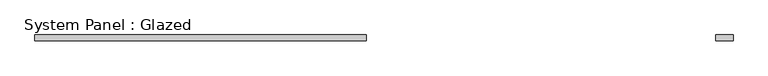
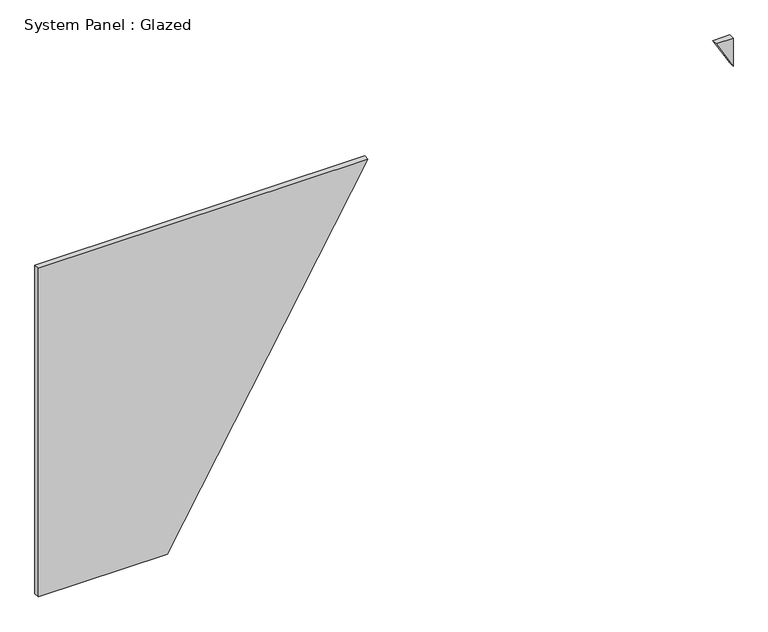
"""IFC4 building model written with IfcOpenShell, lengths in millimetres: plate geometry, System Panel : Glazed."""

from ifc_helpers import new_model, si_unit, frame, origin, place, context, project, spatial, polyline, outline, extrude, source, transform, mapped, element, save


def system_panel_glazed_d44aaf60(model_context):
    return source(origin(), model_context, "Body", "SweptSolid", [
        extrude(outline(polyline([(1500.0, 1426.4508999), (1372.5184302, 1500.0), (1500.0, 1500.0), (1500.0, 1426.4508999)])), frame((0.0, 24.5, 0.0), z_axis=(0.0, 1.0, 0.0), x_axis=(0.0, 0.0, 1.0)), (0.0, 0.0, 1.0), 25.0),
        extrude(outline(polyline([(0.0, -1500.0), (0.0, -943.0853598), (1500.0, -76.4429578), (1500.0, -1500.0), (0.0, -1500.0)])), frame((0.0, 24.5, 0.0), z_axis=(0.0, 1.0, 0.0), x_axis=(0.0, 0.0, 1.0)), (0.0, 0.0, 1.0), 25.0),
    ])


if __name__ == "__main__":
    model = new_model("IFC4")
    model_context = context("Model", 3, world=origin())
    ifc_project = project(units=[si_unit("LENGTHUNIT", "METRE", prefix="MILLI")], contexts=[model_context])
    site = spatial("IfcSite", under=ifc_project)
    building = spatial("IfcBuilding", under=site)
    placement = place(None, origin())
    system_panel_glazed_shape = system_panel_glazed_d44aaf60(model_context)
    element("IfcPlate", 1, ObjectType="System Panel : Glazed", at=placement, inside=building, context=model_context, shape_type="MappedRepresentation", body=[
        mapped(system_panel_glazed_shape, transform((0.0, 0.0, 0.0), x_axis=(1.0, 0.0, 0.0), y_axis=(0.0, 1.0, 0.0), z_axis=(0.0, 0.0, 1.0))),
    ])
    save(model, "model.ifc")

# Revit data of these elements
# Type "System Panel : Glazed"
#   Construction Type Id = "GSP4R"
#   Analytic Construction = "1/8 in Pilkington single glazing"
#   Visual Light Transmittance = 0.9
#   Solar Heat Gain Coefficient = 0.86
#   Heat Transfer Coefficient (U) = 6.7069 W/(m²·K)
#   Define Thermal Properties by = 1
# Element 1 (IfcPlate, "System Panel : Glazed")
#   Materials on its faces: "Glass"
# Materials
#   "Glass": class "Glass", colour RGB 0 128 192, transparency 0.9, Description = "Soda Lime Glass", Cost = 0
